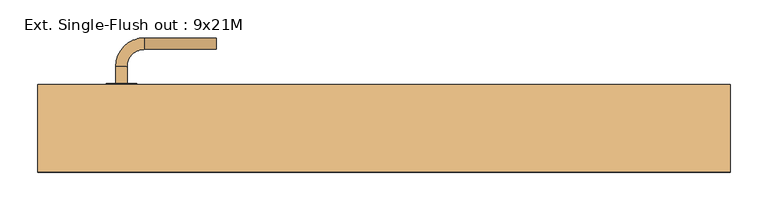
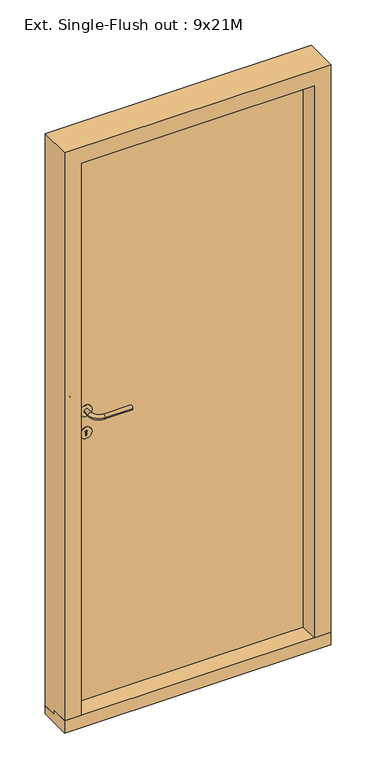
"""IFC4 building model written with IfcOpenShell, lengths in millimetres: door geometry, Ext. Single-Flush out : 9x21M."""

import ifcopenshell
import ifcopenshell.guid

model = None  # the IFC model being written
_history = None  # IfcOwnerHistory: only IFC2X3 demands one
_inside = {}  # id of a spatial element -> (the spatial element, [elements in it])
_under = {}  # id of a project, library or spatial element -> (it, [spatial elements below it])
_declared = {}  # id of a project -> (the project, [libraries it declares])
_typed = {}  # id of a type object -> (the type object, [elements of that type])
_made_of = {}  # id of a material, layer set ... -> (it, [elements and type objects made of it])


def new_model(schema):
    """Start an empty IFC model of exactly this schema.

    Asked for "IFC4X3", IfcOpenShell would pick the latest addendum, in which some entities
    have other attributes; the version numbers below select the first issue.
    IFC2X3 requires an IfcOwnerHistory on every rooted entity: one is made here for all.
    """
    global model, _history
    if schema == "IFC4X3":
        model = ifcopenshell.file(schema_version=(4, 3, 0, 0))
    else:
        model = ifcopenshell.file(schema=schema)
    _inside.clear()
    _under.clear()
    _declared.clear()
    _typed.clear()
    _made_of.clear()
    _history = None
    if model.schema == "IFC2X3":
        org = make("IfcOrganization", Name="unknown")
        user = make(
            "IfcPersonAndOrganization",
            ThePerson=make("IfcPerson", FamilyName="unknown"),
            TheOrganization=org,
        )
        app = make(
            "IfcApplication",
            ApplicationDeveloper=org,
            Version="unknown",
            ApplicationFullName="unknown",
            ApplicationIdentifier="unknown",
        )
        _history = make(
            "IfcOwnerHistory",
            OwningUser=user,
            OwningApplication=app,
            ChangeAction="ADDED",
            CreationDate=0,
        )
    return model


def make(cls, **values):
    """One entity of the class cls with the attributes given. An attribute that is None is left unset."""
    return model.create_entity(
        cls, **{name: value for name, value in values.items() if value is not None}
    )


def rooted(cls, **values):
    """An entity with a GlobalId (a new one), such as an element, a storey or a relation."""
    return make(cls, GlobalId=ifcopenshell.guid.new(), OwnerHistory=_history, **values)


def si_unit(unit_type, name, prefix=None):
    """IfcSIUnit, for example si_unit("LENGTHUNIT", "METRE", prefix="MILLI")."""
    return make("IfcSIUnit", UnitType=unit_type, Prefix=prefix, Name=name)


def assignment(units):
    """IfcUnitAssignment: the units of a project."""
    return None if units is None else make("IfcUnitAssignment", Units=units)


def point(xyz):
    """IfcCartesianPoint."""
    return None if xyz is None else make("IfcCartesianPoint", Coordinates=xyz)


def direction(xyz):
    """IfcDirection."""
    return None if xyz is None else make("IfcDirection", DirectionRatios=xyz)


def frame(location, z_axis=None, x_axis=None):
    """IfcAxis2Placement3D, a coordinate frame: its origin and axes. An axis left out is left unset."""
    return make(
        "IfcAxis2Placement3D",
        Location=point(location),
        Axis=direction(z_axis),
        RefDirection=direction(x_axis),
    )


def frame_2d(location, x_axis=None):
    """IfcAxis2Placement2D, a coordinate frame in the plane: its origin and x axis."""
    return make(
        "IfcAxis2Placement2D", Location=point(location), RefDirection=direction(x_axis)
    )


def origin():
    """The frame at (0, 0, 0) with its axes left unset."""
    return frame((0.0, 0.0, 0.0))


def place(relative_to, where):
    """IfcLocalPlacement: puts the frame where relative to a parent placement (None: the world)."""
    return make(
        "IfcLocalPlacement", PlacementRelTo=relative_to, RelativePlacement=where
    )


def context(
    kind, dimensions, precision=None, world=None, true_north=None, identifier=None
):
    """IfcGeometricRepresentationContext, for example the 3D "Model" context."""
    return make(
        "IfcGeometricRepresentationContext",
        ContextIdentifier=identifier,
        ContextType=kind,
        CoordinateSpaceDimension=dimensions,
        Precision=precision,
        WorldCoordinateSystem=world,
        TrueNorth=true_north,
    )


def project(units=None, contexts=None):
    """IfcProject with its units and contexts."""
    return rooted(
        "IfcProject",
        Name="project",
        RepresentationContexts=contexts,
        UnitsInContext=assignment(units),
    )


def spatial(cls, under=None, at=None, **own):
    """A site, building, storey or space (cls), placed at a placement, below another one or the project."""
    s = rooted(cls, ObjectPlacement=at, **own)
    if under is not None:
        _under.setdefault(under.id(), (under, []))[1].append(s)
    return s


def polyline(points):
    """IfcPolyline through the points."""
    return make("IfcPolyline", Points=[point(p) for p in points])


def circle_curve(where, radius):
    """IfcCircle in the frame where."""
    return make("IfcCircle", Position=where, Radius=radius)


def ellipse_curve(where, semi_axis1, semi_axis2):
    """IfcEllipse in the frame where."""
    return make(
        "IfcEllipse", Position=where, SemiAxis1=semi_axis1, SemiAxis2=semi_axis2
    )


def trimmed(basis, trim1, trim2, sense, master):
    """IfcTrimmedCurve: the piece of a basis curve between two trims."""
    return make(
        "IfcTrimmedCurve",
        BasisCurve=basis,
        Trim1=trim1,
        Trim2=trim2,
        SenseAgreement=sense,
        MasterRepresentation=master,
    )


def segment(curve, same_sense, transition):
    """IfcCompositeCurveSegment."""
    return make(
        "IfcCompositeCurveSegment",
        Transition=transition,
        SameSense=same_sense,
        ParentCurve=curve,
    )


def composite_curve(segments, self_intersect=None):
    """IfcCompositeCurve: segments joined end to end."""
    return make("IfcCompositeCurve", Segments=segments, SelfIntersect=self_intersect)


def outline(outer, holes=None, kind="AREA"):
    """IfcArbitraryClosedProfileDef: a profile drawn as a closed curve; with holes, ...WithVoids."""
    if holes is None:
        return make("IfcArbitraryClosedProfileDef", ProfileType=kind, OuterCurve=outer)
    return make(
        "IfcArbitraryProfileDefWithVoids",
        ProfileType=kind,
        OuterCurve=outer,
        InnerCurves=holes,
    )


def extrude(swept, where, along, depth):
    """IfcExtrudedAreaSolid: the profile swept, set in the frame where, extruded along a direction by depth."""
    return make(
        "IfcExtrudedAreaSolid",
        SweptArea=swept,
        Position=where,
        ExtrudedDirection=direction(along),
        Depth=depth,
    )


def faces_of(points, faces, orient=None, outer=None):
    """IfcFace entities. A face is a list of loops; a loop is a list of indices into points, from 0.

    orient and outer hold one flag for each loop. By default every Orientation is true, the
    first loop of a face is its IfcFaceOuterBound and the others are IfcFaceBound.
    """
    made = []
    for i, loops in enumerate(faces):
        bounds = []
        for j, loop in enumerate(loops):
            is_outer = j == 0 if outer is None else outer[i][j]
            bounds.append(
                make(
                    "IfcFaceOuterBound" if is_outer else "IfcFaceBound",
                    Bound=make("IfcPolyLoop", Polygon=[points[k] for k in loop]),
                    Orientation=True if orient is None else orient[i][j],
                )
            )
        made.append(make("IfcFace", Bounds=bounds))
    return made


def faceted_brep(points, faces, orient=None, outer=None, voids=None):
    """IfcFacetedBrep: a solid bounded by flat faces; with voids (closed shells), ...WithVoids."""
    shared = [point(p) for p in points]
    hull = make("IfcClosedShell", CfsFaces=faces_of(shared, faces, orient, outer))
    if voids is None:
        return make("IfcFacetedBrep", Outer=hull)
    return make(
        "IfcFacetedBrepWithVoids",
        Outer=hull,
        Voids=[
            make(cls, CfsFaces=faces_of(shared, fs, o, b)) for cls, fs, o, b in voids
        ],
    )


def shape(context_of_items, identifier, shape_type, items):
    """IfcShapeRepresentation: the items that make up one representation, for example the "Body"."""
    return make(
        "IfcShapeRepresentation",
        ContextOfItems=context_of_items,
        RepresentationIdentifier=identifier,
        RepresentationType=shape_type,
        Items=items,
    )


def source(mapping_origin, context_of_items, identifier, shape_type, items):
    """IfcRepresentationMap: a shape defined once, which mapped items show again and again."""
    return make(
        "IfcRepresentationMap",
        MappingOrigin=mapping_origin,
        MappedRepresentation=shape(context_of_items, identifier, shape_type, items),
    )


def transform(
    local_origin,
    x_axis=None,
    y_axis=None,
    z_axis=None,
    scale=None,
    scale2=None,
    scale3=None,
    uniform=True,
):
    """IfcCartesianTransformationOperator3D, or its non-uniform kind. x_axis, y_axis, z_axis: its Axis1, 2, 3."""
    if uniform:
        return make(
            "IfcCartesianTransformationOperator3D",
            Axis1=direction(x_axis),
            Axis2=direction(y_axis),
            LocalOrigin=point(local_origin),
            Scale=scale,
            Axis3=direction(z_axis),
        )
    return make(
        "IfcCartesianTransformationOperator3DnonUniform",
        Axis1=direction(x_axis),
        Axis2=direction(y_axis),
        LocalOrigin=point(local_origin),
        Scale=scale,
        Axis3=direction(z_axis),
        Scale2=scale2,
        Scale3=scale3,
    )


def mapped(mapping_source, mapping_target):
    """IfcMappedItem: shows the shape of a source again, moved by a transform."""
    return make(
        "IfcMappedItem", MappingSource=mapping_source, MappingTarget=mapping_target
    )


def made_of(thing, what):
    """Note that an element or type object is made of a material, layer set ...; save() writes the relation."""
    if what is not None:
        _made_of.setdefault(what.id(), (what, []))[1].append(thing)
    return thing


def element(
    cls,
    number,
    at=None,
    inside=None,
    cuts=None,
    type_object=None,
    material=None,
    context=None,
    identifier="Body",
    shape_type=None,
    held_by="IfcProductDefinitionShape",
    body=None,
    shapes=None,
    **own,
):
    """One element of the class cls, such as IfcWall. Its Tag is "e" and its number.

    at: its placement. inside: the storey or other place that contains it. cuts: it is an
    opening in that element (IfcRelVoidsElement). A single representation is given by context,
    identifier, shape_type and body (its items); several are given by shapes. held_by: the class
    of the entity that holds the representations. save() writes the other relations.
    """
    e = rooted(cls, Tag="e%d" % number, ObjectPlacement=at, **own)
    if body is not None:
        shapes = [shape(context, identifier, shape_type, body)]
    if shapes is not None:
        e.Representation = make(held_by, Representations=shapes)
    if inside is not None:
        _inside.setdefault(inside.id(), (inside, []))[1].append(e)
    if cuts is not None:
        rooted(
            "IfcRelVoidsElement", RelatingBuildingElement=cuts, RelatedOpeningElement=e
        )
    if type_object is not None:
        _typed.setdefault(type_object.id(), (type_object, []))[1].append(e)
    return made_of(e, material)


def aggregate(whole, parts):
    """IfcRelAggregates: a whole, such as a stair, and the parts it consists of."""
    return rooted("IfcRelAggregates", RelatingObject=whole, RelatedObjects=parts)


def save(model, path):
    """Write the relations noted so far, then the file.

    IfcRelAggregates (storeys below a building ...), IfcRelContainedInSpatialStructure (elements
    in a storey), IfcRelDefinesByType, IfcRelAssociatesMaterial and IfcRelDeclares: one each for
    every whole, place, type object, material and project.
    """
    for whole, parts in _under.values():
        aggregate(whole, parts)
    for where, things in _inside.values():
        rooted(
            "IfcRelContainedInSpatialStructure",
            RelatedElements=things,
            RelatingStructure=where,
        )
    for kind, things in _typed.values():
        rooted("IfcRelDefinesByType", RelatedObjects=things, RelatingType=kind)
    for what, things in _made_of.values():
        rooted("IfcRelAssociatesMaterial", RelatedObjects=things, RelatingMaterial=what)
    for by, libraries in _declared.values():
        rooted("IfcRelDeclares", RelatingContext=by, RelatedDefinitions=libraries)
    model.write(path)


def plane_surface(at):
    """IfcPlane: the flat surface through the origin of the frame at, square to its z axis."""
    return make("IfcPlane", Position=at)


def cylinder_surface(at, radius):
    """IfcCylindricalSurface: all points at the distance radius from the z axis of the frame at."""
    return make("IfcCylindricalSurface", Position=at, Radius=radius)


def revolved_surface(curve, axis_point, axis_direction):
    """IfcSurfaceOfRevolution: the curve turned about the line through axis_point along axis_direction."""
    return make(
        "IfcSurfaceOfRevolution",
        SweptCurve=make("IfcArbitraryOpenProfileDef", ProfileType="CURVE", Curve=curve),
        AxisPosition=make("IfcAxis1Placement", Location=point(axis_point), Axis=direction(axis_direction)),
    )


def advanced_brep(points, edges, surfaces, faces):
    """IfcAdvancedBrep: a solid bounded by faces that lie on surfaces and meet in shared edges.

    An edge is (start, end): straight between two places in points (the first is 0);
    or (start, end, curve); or (start, end, curve, False) where it runs against its curve.
    A face is (place in surfaces, loops), or (place, loops, False) where it looks against
    its surface's normal. A loop lists edges by number (the first is 1), with a minus sign
    where the edge is run from its end to its start. The first loop is the outer one.
    """
    corners = [point(p) for p in points]
    vertices = [make("IfcVertexPoint", VertexGeometry=c) for c in corners]
    made = []
    for start, end, *more in edges:
        made.append(
            make(
                "IfcEdgeCurve",
                EdgeStart=vertices[start],
                EdgeEnd=vertices[end],
                EdgeGeometry=more[0] if more else make("IfcPolyline", Points=[corners[start], corners[end]]),
                SameSense=more[1] if len(more) > 1 else True,
            )
        )
    hull = []
    for where, loops, *sense in faces:
        bounds = []
        for j, loop in enumerate(loops):
            ring = [make("IfcOrientedEdge", EdgeElement=made[abs(k) - 1], Orientation=k > 0) for k in loop]
            bounds.append(
                make(
                    "IfcFaceOuterBound" if j == 0 else "IfcFaceBound",
                    Bound=make("IfcEdgeLoop", EdgeList=ring),
                    Orientation=True,
                )
            )
        hull.append(make("IfcAdvancedFace", Bounds=bounds, FaceSurface=surfaces[where], SameSense=sense[0] if sense else True))
    return make("IfcAdvancedBrep", Outer=make("IfcClosedShell", CfsFaces=hull))


def ext_single_flush_out_9x21m_755ac03d(model_context):
    return source(origin(), model_context, "Body", "SolidModel", [
        extrude(outline(composite_curve([segment(trimmed(circle_curve(frame_2d((1090.0, -346.0)), 20.0), [point((1070.0, -346.0))], [point((1110.0, -346.0))], False, "CARTESIAN"), True, "CONTINUOUS"), segment(trimmed(circle_curve(frame_2d((1090.0, -346.0)), 20.0), [point((1110.0, -346.0))], [point((1070.0, -346.0))], False, "CARTESIAN"), True, "CONTINUOUS")], self_intersect=False)), frame((0.0, 184.0, 0.0), z_axis=(0.0, 1.0, 0.0), x_axis=(0.0, 0.0, 1.0)), (0.0, 0.0, 1.0), 2.0),
        advanced_brep(
        [(-353.5, 186.0, 1090.0), (-338.5, 186.0, 1090.0), (-353.5, 208.5, 1090.0), (-338.5, 208.5, 1090.0), (-316.0, 231.0, 1090.0), (-316.0, 246.0, 1090.0), (-221.0, 246.0, 1090.0), (-221.0, 231.0, 1090.0)],
        [
            (0, 1, circle_curve(frame((-346.0, 186.0, 1090.0), z_axis=(0.0, -1.0, 0.0), x_axis=(1.0, 0.0, 0.0)), 7.5)),
            (1, 0, circle_curve(frame((-346.0, 186.0, 1090.0), z_axis=(0.0, -1.0, 0.0), x_axis=(1.0, 0.0, 0.0)), 7.5)),
            (0, 2),
            (2, 3, circle_curve(frame((-346.0, 208.5, 1090.0), z_axis=(0.0, -1.0, 0.0), x_axis=(1.0, 0.0, 0.0)), 7.5)),
            (3, 1),
            (3, 2, circle_curve(frame((-346.0, 208.5, 1090.0), z_axis=(0.0, -1.0, 0.0), x_axis=(1.0, 0.0, 0.0)), 7.5)),
            (4, 3, circle_curve(frame((-316.0, 208.5, 1090.0), z_axis=(0.0, 0.0, 1.0), x_axis=(-1.0, 0.0, 0.0)), 22.5)),
            (2, 5, circle_curve(frame((-316.0, 208.5, 1090.0), z_axis=(0.0, 0.0, -1.0), x_axis=(-1.0, 0.0, 0.0)), 37.5)),
            (5, 4, circle_curve(frame((-316.0, 238.5, 1090.0), z_axis=(-1.0, 0.0, 0.0), x_axis=(0.0, -1.0, 0.0)), 7.5)),
            (4, 5, circle_curve(frame((-316.0, 238.5, 1090.0), z_axis=(-1.0, 0.0, 0.0), x_axis=(0.0, -1.0, 0.0)), 7.5)),
            (5, 6),
            (6, 7, circle_curve(frame((-221.0, 238.5, 1090.0), z_axis=(-1.0, 0.0, 0.0), x_axis=(0.0, -1.0, 0.0)), 7.5)),
            (7, 4),
            (7, 6, circle_curve(frame((-221.0, 238.5, 1090.0), z_axis=(-1.0, 0.0, 0.0), x_axis=(0.0, -1.0, 0.0)), 7.5)),
        ],
        [
            plane_surface(frame((-346.0, 186.0, 1090.0), z_axis=(0.0, -1.0, 0.0), x_axis=(0.0, 0.0, -1.0))),
            cylinder_surface(frame((-346.0, 186.0, 1090.0), z_axis=(0.0, -1.0, 0.0), x_axis=(1.0, 0.0, 0.0)), 7.5),
            revolved_surface(trimmed(ellipse_curve(frame((-346.0, 208.5, 1090.0), z_axis=(0.0, -1.0, 0.0), x_axis=(1.0, 0.0, 0.0)), 7.5, 7.5), [point((-353.5, 208.5, 1090.0))], [point((-338.5, 208.5, 1090.0))], True, "CARTESIAN"), (-316.0, 208.5, 1090.0), (0.0, 0.0, -1.0)),
            revolved_surface(trimmed(ellipse_curve(frame((-346.0, 208.5, 1090.0), z_axis=(0.0, -1.0, 0.0), x_axis=(1.0, 0.0, 0.0)), 7.5, 7.5), [point((-338.5, 208.5, 1090.0))], [point((-353.5, 208.5, 1090.0))], True, "CARTESIAN"), (-316.0, 208.5, 1090.0), (0.0, 0.0, -1.0)),
            cylinder_surface(frame((-316.0, 238.5, 1090.0), z_axis=(-1.0, 0.0, 0.0), x_axis=(0.0, -1.0, 0.0)), 7.5),
            plane_surface(frame((-221.0, 238.5, 1090.0), z_axis=(1.0, 0.0, 0.0), x_axis=(0.0, 0.0, -1.0))),
        ],
        [
            (0, [[1, 2]]),
            (1, [[-1, 3, 4, 5]]),
            (1, [[-2, -5, 6, -3]]),
            (2, [[7, -4, 8, 9]]),
            (3, [[-8, -6, -7, 10]]),
            (4, [[-9, 11, 12, 13]]),
            (4, [[-10, -13, 14, -11]]),
            (5, [[-14, -12]]),
        ],
    ),
        extrude(outline(composite_curve([segment(trimmed(circle_curve(frame_2d((1010.0, -346.0)), 20.0), [point((990.0, -346.0))], [point((1030.0, -346.0))], False, "CARTESIAN"), True, "CONTINUOUS"), segment(trimmed(circle_curve(frame_2d((1010.0, -346.0)), 20.0), [point((1030.0, -346.0))], [point((990.0, -346.0))], False, "CARTESIAN"), True, "CONTINUOUS")], self_intersect=False), holes=[composite_curve([segment(trimmed(circle_curve(frame_2d((1015.0, -346.0)), 3.0), [point((1012.4019238, -347.5))], [point((1012.4019238, -344.5))], True, "CARTESIAN"), True, "CONTINUOUS"), segment(polyline([(1012.4019238, -344.5), (1000.0, -344.5), (1000.0, -347.5), (1012.4019238, -347.5)]), True, "CONTINUOUS")], self_intersect=False)]), frame((0.0, 184.0, 0.0), z_axis=(0.0, 1.0, 0.0), x_axis=(0.0, 0.0, 1.0)), (0.0, 0.0, 1.0), 2.0),
        extrude(outline(composite_curve([segment(trimmed(circle_curve(frame_2d((1090.0, -346.0)), 20.0), [point((1070.0, -346.0))], [point((1110.0, -346.0))], False, "CARTESIAN"), True, "CONTINUOUS"), segment(trimmed(circle_curve(frame_2d((1090.0, -346.0)), 20.0), [point((1110.0, -346.0))], [point((1070.0, -346.0))], False, "CARTESIAN"), True, "CONTINUOUS")], self_intersect=False)), frame((0.0, 132.0, 0.0), z_axis=(0.0, 1.0, 0.0), x_axis=(0.0, 0.0, 1.0)), (0.0, 0.0, 1.0), 2.0),
        advanced_brep(
        [(-353.5, 132.0, 1090.0), (-338.5, 132.0, 1090.0), (-338.5, 109.5, 1090.0), (-353.5, 109.5, 1090.0), (-316.0, 87.0, 1090.0), (-316.0, 72.0, 1090.0), (-221.0, 87.0, 1090.0), (-221.0, 72.0, 1090.0)],
        [
            (0, 1, circle_curve(frame((-346.0, 132.0, 1090.0), z_axis=(0.0, 1.0, 0.0), x_axis=(1.0, 0.0, 0.0)), 7.5)),
            (1, 0, circle_curve(frame((-346.0, 132.0, 1090.0), z_axis=(0.0, 1.0, 0.0), x_axis=(1.0, 0.0, 0.0)), 7.5)),
            (1, 2),
            (2, 3, circle_curve(frame((-346.0, 109.5, 1090.0), z_axis=(0.0, 1.0, 0.0), x_axis=(1.0, 0.0, 0.0)), 7.5)),
            (3, 0),
            (3, 2, circle_curve(frame((-346.0, 109.5, 1090.0), z_axis=(0.0, 1.0, 0.0), x_axis=(1.0, 0.0, 0.0)), 7.5)),
            (4, 5, circle_curve(frame((-316.0, 79.5, 1090.0), z_axis=(-1.0, 0.0, 0.0), x_axis=(0.0, 1.0, 0.0)), 7.5)),
            (5, 3, circle_curve(frame((-316.0, 109.5, 1090.0), z_axis=(0.0, 0.0, -1.0), x_axis=(-1.0, 0.0, 0.0)), 37.5)),
            (2, 4, circle_curve(frame((-316.0, 109.5, 1090.0), z_axis=(0.0, 0.0, 1.0), x_axis=(-1.0, 0.0, 0.0)), 22.5)),
            (5, 4, circle_curve(frame((-316.0, 79.5, 1090.0), z_axis=(-1.0, 0.0, 0.0), x_axis=(0.0, 1.0, 0.0)), 7.5)),
            (4, 6),
            (6, 7, circle_curve(frame((-221.0, 79.5, 1090.0), z_axis=(-1.0, 0.0, 0.0), x_axis=(0.0, 1.0, 0.0)), 7.5)),
            (7, 5),
            (7, 6, circle_curve(frame((-221.0, 79.5, 1090.0), z_axis=(-1.0, 0.0, 0.0), x_axis=(0.0, 1.0, 0.0)), 7.5)),
        ],
        [
            plane_surface(frame((-346.0, 132.0, 1090.0), z_axis=(0.0, 1.0, 0.0), x_axis=(0.0, 0.0, -1.0))),
            cylinder_surface(frame((-346.0, 132.0, 1090.0), z_axis=(0.0, 1.0, 0.0), x_axis=(1.0, 0.0, 0.0)), 7.5),
            revolved_surface(trimmed(ellipse_curve(frame((-346.0, 109.5, 1090.0), z_axis=(0.0, -1.0, 0.0), x_axis=(1.0, 0.0, 0.0)), 7.5, 7.5), [point((-353.5, 109.5, 1090.0))], [point((-338.5, 109.5, 1090.0))], True, "CARTESIAN"), (-316.0, 109.5, 1090.0), (0.0, 0.0, -1.0)),
            revolved_surface(trimmed(ellipse_curve(frame((-346.0, 109.5, 1090.0), z_axis=(0.0, -1.0, 0.0), x_axis=(1.0, 0.0, 0.0)), 7.5, 7.5), [point((-338.5, 109.5, 1090.0))], [point((-353.5, 109.5, 1090.0))], True, "CARTESIAN"), (-316.0, 109.5, 1090.0), (0.0, 0.0, -1.0)),
            cylinder_surface(frame((-316.0, 79.5, 1090.0), z_axis=(-1.0, 0.0, 0.0), x_axis=(0.0, 1.0, 0.0)), 7.5),
            plane_surface(frame((-221.0, 79.5, 1090.0), z_axis=(1.0, 0.0, 0.0), x_axis=(0.0, 0.0, -1.0))),
        ],
        [
            (0, [[1, 2]]),
            (1, [[3, 4, 5, -2]]),
            (1, [[-5, 6, -3, -1]]),
            (2, [[7, 8, -4, 9]]),
            (3, [[10, -9, -6, -8]]),
            (4, [[11, 12, 13, -7]]),
            (4, [[-13, 14, -11, -10]]),
            (5, [[-12, -14]]),
        ],
    ),
        extrude(outline(composite_curve([segment(trimmed(circle_curve(frame_2d((1010.0, -346.0)), 20.0), [point((990.0, -346.0))], [point((1030.0, -346.0))], False, "CARTESIAN"), True, "CONTINUOUS"), segment(trimmed(circle_curve(frame_2d((1010.0, -346.0)), 20.0), [point((1030.0, -346.0))], [point((990.0, -346.0))], False, "CARTESIAN"), True, "CONTINUOUS")], self_intersect=False), holes=[composite_curve([segment(trimmed(circle_curve(frame_2d((1015.0, -346.0)), 3.0), [point((1012.4019238, -347.5))], [point((1012.4019238, -344.5))], True, "CARTESIAN"), True, "CONTINUOUS"), segment(polyline([(1012.4019238, -344.5), (1000.0, -344.5), (1000.0, -347.5), (1012.4019238, -347.5)]), True, "CONTINUOUS")], self_intersect=False)]), frame((0.0, 132.0, 0.0), z_axis=(0.0, 1.0, 0.0), x_axis=(0.0, 0.0, 1.0)), (0.0, 0.0, 1.0), 2.0),
        extrude(outline(polyline([(-414.0, 184.0), (414.0, 184.0), (414.0, 134.0), (-414.0, 134.0), (-414.0, 184.0)])), frame((0.0, 0.0, 30.0), z_axis=(0.0, 0.0, 1.0), x_axis=(1.0, 0.0, 0.0)), (0.0, 0.0, 1.0), 2028.0),
        faceted_brep([(414.0, 184.0, 2058.0), (-414.0, 184.0, 2058.0), (-414.0, 184.0, 30.0), (-456.0, 184.0, 30.0), (-456.0, 184.0, 2100.0), (456.0, 184.0, 2100.0), (456.0, 184.0, 30.0), (414.0, 184.0, 30.0), (-414.0, 134.0, 2058.0), (-414.0, 134.0, 45.0), (-414.0, 134.0, 30.0), (456.0, 134.0, 30.0), (414.0, 134.0, 30.0), (-456.0, 134.0, 30.0), (-456.0, 69.0, 2100.0), (-456.0, 134.0, 45.0), (-456.0, 69.0, 45.0), (456.0, 69.0, 2100.0), (456.0, 69.0, 45.0), (456.0, 134.0, 45.0), (414.0, 134.0, 2058.0), (414.0, 134.0, 45.0), (-399.0, 69.0, 45.0), (-399.0, 69.0, 2043.0), (399.0, 69.0, 2043.0), (399.0, 69.0, 45.0), (399.0, 134.0, 45.0), (-399.0, 134.0, 45.0), (-399.0, 134.0, 2043.0), (399.0, 134.0, 2043.0)], [[[0, 1, 2, 3, 4, 5, 6, 7]], [[1, 8, 9, 10, 2]], [[11, 12, 7, 6]], [[10, 13, 3, 2]], [[14, 4, 3, 13, 15, 16]], [[5, 17, 18, 19, 11, 6]], [[20, 0, 7, 12, 21]], [[17, 14, 16, 22, 23, 24, 25, 18]], [[21, 19, 18, 25, 26]], [[15, 9, 27, 22, 16]], [[19, 21, 12, 11]], [[9, 15, 13, 10]], [[28, 23, 22, 27]], [[24, 29, 26, 25]], [[29, 28, 27, 9, 8, 20, 21, 26]], [[5, 4, 14, 17]], [[24, 23, 28, 29]], [[1, 0, 20, 8]]]),
        extrude(outline(polyline([(184.0, 30.0), (184.0, 0.0), (69.0, 0.0), (69.0, 45.0), (134.0, 45.0), (134.0, 30.0), (184.0, 30.0)])), frame((-456.0, 0.0, 0.0), z_axis=(1.0, 0.0, 0.0), x_axis=(0.0, 1.0, 0.0)), (0.0, 0.0, 1.0), 912.0),
    ])


if __name__ == "__main__":
    model = new_model("IFC4")
    model_context = context("Model", 3, world=origin())
    ifc_project = project(units=[si_unit("LENGTHUNIT", "METRE", prefix="MILLI")], contexts=[model_context])
    site = spatial("IfcSite", under=ifc_project)
    building = spatial("IfcBuilding", under=site)
    placement = place(None, origin())
    ext_single_flush_out_9x21m_shape = ext_single_flush_out_9x21m_755ac03d(model_context)
    element("IfcDoor", 1, ObjectType="Ext. Single-Flush out : 9x21M", at=placement, inside=building, context=model_context, shape_type="MappedRepresentation", body=[
        mapped(ext_single_flush_out_9x21m_shape, transform((0.0, 0.0, 0.0), x_axis=(1.0, 0.0, 0.0), y_axis=(0.0, 1.0, 0.0), z_axis=(0.0, 0.0, 1.0))),
    ])
    save(model, "model.ifc")

# Revit data of these elements
# Project information
#   Client Name = "Test Project"
#   Project Address = "Enter address here"
#   Project Number = "Number"
#   Current Version = "0.0.0"
#   SR Document GUID = "3eb9317e-835d-4f79-8926-4d15b96bc824"
# Type "Ext. Single-Flush out : 9x21M"
#   Type Mark = "63"
#   Sound Rating = ""
#   Opening Side [instance default] = "out"
#   Hinge Side [instance default] = ""
#   Creator Organization [instance default] = "© Danish Educational Content"
#   Creator Name [instance default] = "© Erik Falck Jørgensen"
#   Creator Build [instance default] = "2017.0301.0"
#   Analytic Construction = "<None>"
#   length#6 = -50 mm
#   length#4 = 120 mm
#   length#5 = 912 mm
#   length#3 = 30 mm
#   length#2 = 57 mm
#   length#1 = 0 mm
#   Thickness = 50 mm
#   Seal Width = 12 mm
#   Rough Width = 912 mm
#   Rough Height = 2100 mm
#   Rebate Depth = 50 mm
#   Rabbet Width = 15 mm
#   Rabbet Depth = 50 mm
#   Height = 2088 mm
#   Width = 888 mm
#   Handle From Side = 110 mm
#   Handle From Bottom = 1090 mm
#   Exterior Direction [instance default] = 0.00°
#   Case Depth = 115 mm
#   Case Width = 45 mm
#   Threshold = yes
#   Sealing = no
#   Hinging = yes
#   Wall Closure = 1
#   Function = 1
#   Panel = none
#   Handle Finish = none
#   Handle = element 632149
#   Case/Transom = none
#   Assembly Code = ""
# Element 1 (IfcDoor, "Ext. Single-Flush out : 9x21M")
#   Materials on its faces: "Stainless Steel, Polished", "Default Frame/Mullion (Interior/Exterior)", "Default Door Panel (Exterior/Interior)"
# Materials
#   "Stainless Steel, Polished": class "Metal", colour RGB 180 180 180, transparency 0, Description = "Rustfri stål, poleret", Cost = 0
#   "Default Frame/Mullion (Interior/Exterior)": class "Generic", colour RGB 205 205 205, transparency 0, Description = "Udefineret karm/ramme materiale", Cost = 0
#   "Default Door Panel (Exterior/Interior)": class "Generic", colour RGB 205 205 205, transparency 0, Description = "Udefineret dørplade materiale", Cost = 0
